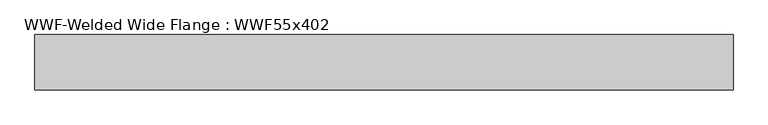
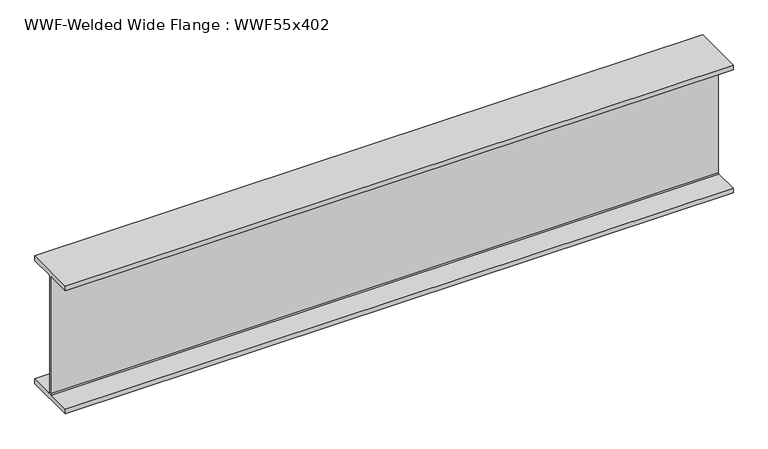
"""IFC4 building model written with IfcOpenShell, lengths in millimetres: beam geometry, WWF-Welded Wide Flange : WWF55x402."""

from ifc_helpers import new_model, si_unit, frame, origin, place, context, project, spatial, polyline, outline, extrude, source, transform, mapped, element, save


def wwf_welded_wide_flange_wwf55x402_6292d54f(model_context):
    return source(origin(), model_context, "Body", "SweptSolid", [
        extrude(outline(polyline([(274.955, -649.986), (274.955, -700.024), (-274.955, -700.024), (-274.955, -649.986), (-19.05, -649.986), (-8.001, -638.937), (-8.001, 638.937), (-19.05, 649.986), (-274.955, 649.986), (-274.955, 700.024), (274.955, 700.024), (274.955, 649.986), (19.05, 649.986), (8.001, 638.937), (8.001, -638.937), (19.05, -649.986), (274.955, -649.986)])), frame((-3472.2230903, 0.0, 0.0), z_axis=(1.0, 0.0, 0.0), x_axis=(0.0, 1.0, 0.0)), (0.0, 0.0, 1.0), 6931.7461799),
    ])


if __name__ == "__main__":
    model = new_model("IFC4")
    model_context = context("Model", 3, world=origin())
    ifc_project = project(units=[si_unit("LENGTHUNIT", "METRE", prefix="MILLI")], contexts=[model_context])
    site = spatial("IfcSite", under=ifc_project)
    building = spatial("IfcBuilding", under=site)
    placement = place(None, origin())
    wwf_welded_wide_flange_wwf55x402_shape = wwf_welded_wide_flange_wwf55x402_6292d54f(model_context)
    element("IfcBeam", 1, ObjectType="WWF-Welded Wide Flange : WWF55x402", at=placement, inside=building, context=model_context, shape_type="MappedRepresentation", body=[
        mapped(wwf_welded_wide_flange_wwf55x402_shape, transform((0.0, 0.0, 0.0), x_axis=(1.0, 0.0, 0.0), y_axis=(0.0, 1.0, 0.0), z_axis=(0.0, 0.0, 1.0))),
    ])
    save(model, "model.ifc")

# Revit data of these elements
# Type "WWF-Welded Wide Flange : WWF55x402"
#   Assembly Code = "B10"
#   Nominal d = "12"
#   W = 402
#   Length [instance default] = 1524 mm
#   bf = 549.91 mm
#   d = 1400.048 mm
#   k = 19.05 mm
#   tf = 50.038 mm
#   tw = 16.002 mm
#   A = 0.0761289 m²
#   Structural Material [instance default] = Steel ASTM A572
# Element 1 (IfcBeam, "WWF-Welded Wide Flange : WWF55x402")
#   Structural Material = Metal - Steel 43-275
#   Materials on its faces: "Metal - Steel 43-275"
# Materials
#   "Steel ASTM A572": class "Metal", colour RGB 247 247 247, transparency 0, Description = "Structural steel, high strength low alloy, ASTM - A572 - 50", Cost = 0
#   "Metal - Steel 43-275": class "Metal", colour RGB 247 247 247, transparency 0, Cost = 0
